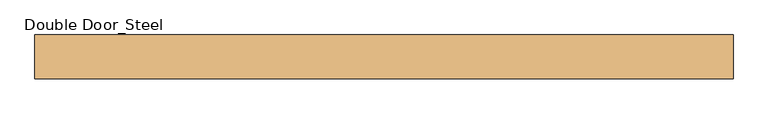
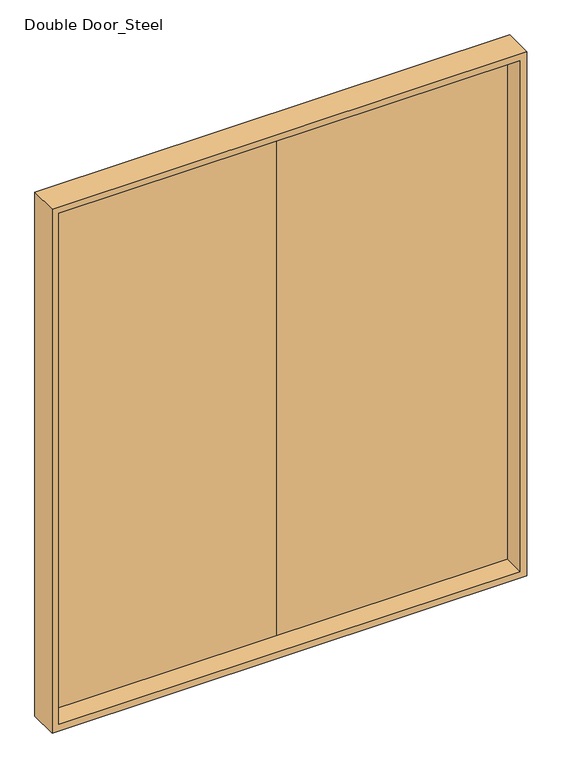
"""IFC4 building model written with IfcOpenShell, lengths in millimetres: door geometry, Double Door_Steel : H_DR_AR_B12_Double Door_Steel_W2400xH2800."""

from ifc_helpers import new_model, si_unit, frame, origin, place, context, project, spatial, polyline, outline, extrude, faceted_brep, source, transform, mapped, element, save


def double_door_steel_3c62acbf(model_context):
    return source(origin(), model_context, "Body", "SolidModel", [
        extrude(outline(polyline([(1180.0, 35.0), (0.0, 35.0), (0.0, 75.0), (1180.0, 75.0), (1180.0, 35.0)])), frame((0.0, 0.0, 20.0), z_axis=(0.0, 0.0, 1.0), x_axis=(1.0, 0.0, 0.0)), (0.0, 0.0, 1.0), 2760.0),
        extrude(outline(polyline([(0.0, 35.0), (-1180.0, 35.0), (-1180.0, 75.0), (0.0, 75.0), (0.0, 35.0)])), frame((0.0, 0.0, 20.0), z_axis=(0.0, 0.0, 1.0), x_axis=(1.0, 0.0, 0.0)), (0.0, 0.0, 1.0), 2760.0),
        faceted_brep([(1200.0, -75.0, 2800.0), (1200.0, 75.0, 2800.0), (-1200.0, 75.0, 2800.0), (-1200.0, -75.0, 2800.0), (1165.0, 35.0, 2765.0), (1165.0, -75.0, 2765.0), (-1165.0, -75.0, 2765.0), (-1165.0, 35.0, 2765.0), (1180.0, 75.0, 2780.0), (1180.0, 35.0, 2780.0), (-1180.0, 35.0, 2780.0), (-1180.0, 75.0, 2780.0), (-1200.0, 75.0, 0.0), (-1200.0, -75.0, 0.0), (-1165.0, -75.0, 35.0), (-1165.0, 35.0, 35.0), (-1180.0, 35.0, 20.0), (-1180.0, 75.0, 20.0), (1200.0, 75.0, 0.0), (1180.0, 75.0, 20.0), (1200.0, -75.0, 0.0), (1165.0, -75.0, 35.0), (1165.0, 35.0, 35.0), (1180.0, 35.0, 20.0)], [[[0, 1, 2, 3]], [[4, 5, 6, 7]], [[8, 9, 10, 11]], [[3, 2, 12, 13]], [[7, 6, 14, 15]], [[11, 10, 16, 17]], [[18, 12, 2, 1], [8, 11, 17, 19]], [[13, 12, 18, 20]], [[0, 3, 13, 20], [21, 14, 6, 5]], [[15, 14, 21, 22]], [[23, 16, 10, 9], [4, 7, 15, 22]], [[17, 16, 23, 19]], [[20, 18, 1, 0]], [[22, 21, 5, 4]], [[19, 23, 9, 8]]]),
    ])


if __name__ == "__main__":
    model = new_model("IFC4")
    model_context = context("Model", 3, world=origin())
    ifc_project = project(units=[si_unit("LENGTHUNIT", "METRE", prefix="MILLI")], contexts=[model_context])
    site = spatial("IfcSite", under=ifc_project)
    building = spatial("IfcBuilding", under=site)
    placement = place(None, origin())
    double_door_steel_shape = double_door_steel_3c62acbf(model_context)
    element("IfcDoor", 1, ObjectType="Double Door_Steel : H_DR_AR_B12_Double Door_Steel_W2400xH2800", at=placement, inside=building, context=model_context, shape_type="MappedRepresentation", body=[
        mapped(double_door_steel_shape, transform((0.0, 0.0, 0.0), x_axis=(1.0, 0.0, 0.0), y_axis=(0.0, 1.0, 0.0), z_axis=(0.0, 0.0, 1.0))),
    ])
    save(model, "model.ifc")

# Revit data of these elements
# Type "Double Door_Steel : H_DR_AR_B12_Double Door_Steel_W2400xH2800"
#   Type Mark = "429"
#   프레임 = ""
#   철물 = ""
#   유리/마감 = ""
#   위치/개소 = ""
#   부호 = "1/SD"
#   문번호 = ""
#   문기호 = "SD"
#   Analytic Construction = "<None>"
#   Height = 2800 mm
#   Width = 2400 mm
#   Define Thermal Properties by = 1
#   문 틀 = none
#   문 = none
#   Function = (empty or 0)
#   Assembly Code = ""
#   Wall Closure = (empty or 0)
